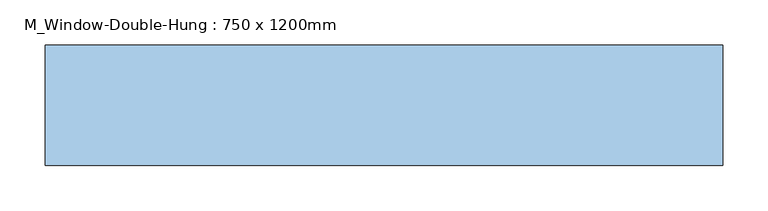
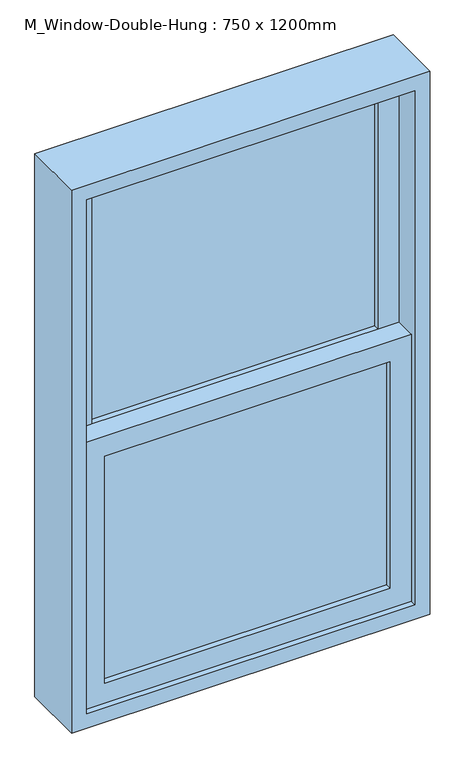
"""IFC4 building model written with IfcOpenShell, lengths in millimetres: window geometry, M_Window-Double-Hung : 750 x 1200mm."""

from ifc_helpers import new_model, si_unit, frame, origin, place, context, project, spatial, polyline, outline, extrude, source, transform, mapped, element, save


def m_window_double_hung_750_x_1200mm_e7ea5f28(model_context):
    return source(origin(), model_context, "Body", "SweptSolid", [
        extrude(outline(polyline([(298.8, -669.85), (298.8, -676.2), (-298.8, -676.2), (-298.8, -669.85), (298.8, -669.85)])), frame((0.0, 0.0, 990.6), z_axis=(0.0, 0.0, 1.0), x_axis=(1.0, 0.0, 0.0)), (0.0, 0.0, 1.0), 501.575),
        extrude(outline(polyline([(-298.8, -682.55), (298.8, -682.55), (298.8, -688.9), (-298.8, -688.9), (-298.8, -682.55)])), frame((0.0, 0.0, 990.6), z_axis=(0.0, 0.0, 1.0), x_axis=(1.0, 0.0, 0.0)), (0.0, 0.0, 1.0), 501.575),
        extrude(outline(polyline([(298.8, -625.4), (298.8, -631.75), (-298.8, -631.75), (-298.8, -625.4), (298.8, -625.4)])), frame((0.0, 0.0, 1536.625), z_axis=(0.0, 0.0, 1.0), x_axis=(1.0, 0.0, 0.0)), (0.0, 0.0, 1.0), 501.575),
        extrude(outline(polyline([(-298.8, -638.1), (298.8, -638.1), (298.8, -644.45), (-298.8, -644.45), (-298.8, -638.1)])), frame((0.0, 0.0, 1536.625), z_axis=(0.0, 0.0, 1.0), x_axis=(1.0, 0.0, 0.0)), (0.0, 0.0, 1.0), 501.575),
        extrude(outline(polyline([(1536.625, -343.25), (946.15, -343.25), (946.15, 343.25), (1536.625, 343.25), (1536.625, -343.25)]), holes=[polyline([(1492.175, 298.8), (990.6, 298.8), (990.6, -298.8), (1492.175, -298.8), (1492.175, 298.8)])]), frame((0.0, -701.6, 0.0), z_axis=(0.0, 1.0, 0.0), x_axis=(0.0, 0.0, 1.0)), (0.0, 0.0, 1.0), 44.45),
        extrude(outline(polyline([(2082.65, -343.25), (1492.175, -343.25), (1492.175, 343.25), (2082.65, 343.25), (2082.65, -343.25)]), holes=[polyline([(2038.2, 298.8), (1536.625, 298.8), (1536.625, -298.8), (2038.2, -298.8), (2038.2, 298.8)])]), frame((0.0, -657.15, 0.0), z_axis=(0.0, 1.0, 0.0), x_axis=(0.0, 0.0, 1.0)), (0.0, 0.0, 1.0), 44.45),
        extrude(outline(polyline([(2114.4, -375.0), (914.4, -375.0), (914.4, 375.0), (2114.4, 375.0), (2114.4, -375.0)]), holes=[polyline([(2082.65, 343.25), (946.15, 343.25), (946.15, -343.25), (2082.65, -343.25), (2082.65, 343.25)])]), frame((0.0, -714.3, 0.0), z_axis=(0.0, 1.0, 0.0), x_axis=(0.0, 0.0, 1.0)), (0.0, 0.0, 1.0), 133.35),
    ])


if __name__ == "__main__":
    model = new_model("IFC4")
    model_context = context("Model", 3, world=origin())
    ifc_project = project(units=[si_unit("LENGTHUNIT", "METRE", prefix="MILLI")], contexts=[model_context])
    site = spatial("IfcSite", under=ifc_project)
    building = spatial("IfcBuilding", under=site)
    placement = place(None, origin())
    m_window_double_hung_750_x_1200mm_shape = m_window_double_hung_750_x_1200mm_e7ea5f28(model_context)
    element("IfcWindow", 1, ObjectType="M_Window-Double-Hung : 750 x 1200mm", at=placement, inside=building, context=model_context, shape_type="MappedRepresentation", body=[
        mapped(m_window_double_hung_750_x_1200mm_shape, transform((0.0, 0.0, 0.0), x_axis=(1.0, 0.0, 0.0), y_axis=(0.0, 1.0, 0.0), z_axis=(0.0, 0.0, 1.0))),
    ])
    save(model, "model.ifc")

# Revit data of these elements
# Type "M_Window-Double-Hung : 750 x 1200mm"
#   Type Mark = "22"
#   Fire Rating = "0.5h"
#   Construction Type Id = "DG-DR"
#   Assembly Code = "B2020100"
#   Analytic Construction = "Double glazing - domestic"
#   Wall Thickness [instance default] = 150 mm
#   Window Inset [instance default] = 0 mm
#   Visual Light Transmittance = 0.81
#   Thermal Resistance (R) = 0.319569 (m²·K)/W
#   Solar Heat Gain Coefficient = 0.76
#   Muntin Width = 597.6 mm
#   Muntin Height = 501.575 mm
#   Interior Wall Closure [instance default] = 35.7 mm
#   Rough Width = 765 mm
#   Rough Height = 1215 mm
#   Frame Extension [instance default] = 31.75 mm
#   Exterior Wall Closure [instance default] = 12.7 mm
#   Extension Jamb [instance default] = 35.7 mm
#   Heat Transfer Coefficient (U) = 3.12929 W/(m²·K)
#   Height = 1200 mm
#   Width = 750 mm
#   Define Thermal Properties by = 1
#   Top Muntin Visibility = yes
#   Indicator Visibility [instance default] = yes
#   Extension Jamb Visibility [instance default] = yes
#   Interior Trim Visibility [instance default] = yes
#   Exterior Trim Visibility [instance default] = yes
#   Define Thermal Properties by = 1
#   Bottom Muntin Visibility = yes
#   Muntin Pattern = M_Muntin Pattern_2x2 : M_Muntin Pattern_2x2
#   Interior Trim Material = Wood - Stained
#   Interior Trim = M_Trim-Window-Interior-Flat : Picture Frame
#   Exterior Trim Material = Clad - White
#   Exterior Trim = M_Trim-Window-Exterior-Flat : with Sill
#   Glass Panel Material = Glass
#   Exterior Frame Material = Clad - White
#   Interior Frame Material = Wood - Stained
#   Wall Closure = (empty or 0)
# Element 1 (IfcWindow, "M_Window-Double-Hung : 750 x 1200mm")
#   Wall Thickness = 200 mm
#   Window Inset = 700 mm
#   Interior Wall Closure = 60 mm
#   Exterior Wall Closure = 50 mm
#   Extension Jamb = 25.4 mm
#   Indicator Visibility = no
#   Extension Jamb Visibility = no
#   Interior Trim Visibility = no
#   Exterior Trim Visibility = no
#   Materials on its faces: "Wood - Stained", "Glass", "Clad - White"
# Materials
#   "Wood - Stained": class "Wood", colour RGB 224 178 126, transparency 0, Cost = 0
#   "Clad - White": class "Wood", colour RGB 242 242 238, transparency 0, Cost = 0
#   "Glass": class "Glass", colour RGB 0 128 192, transparency 0.9, Description = "Soda Lime Glass", Cost = 0
